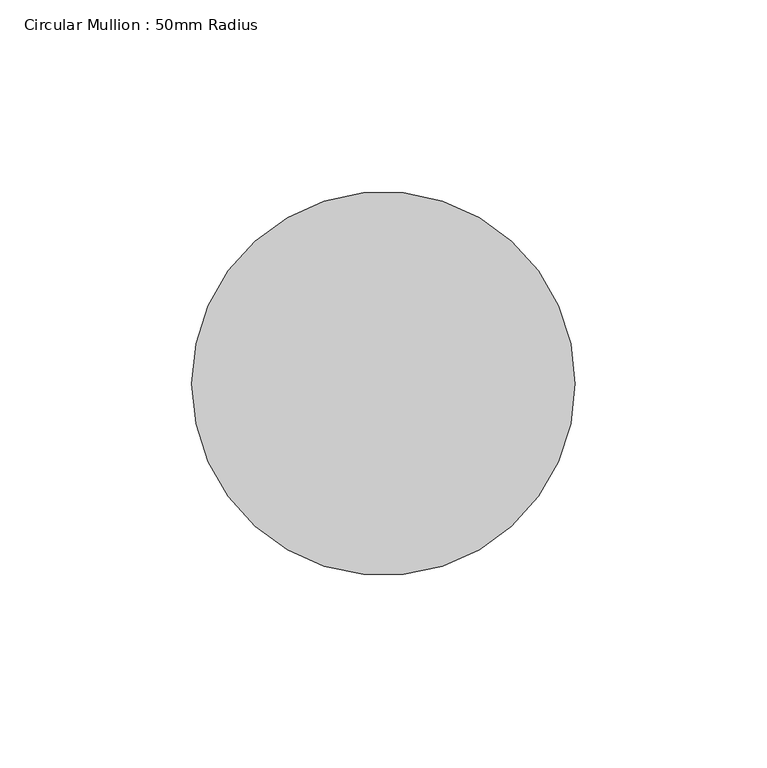
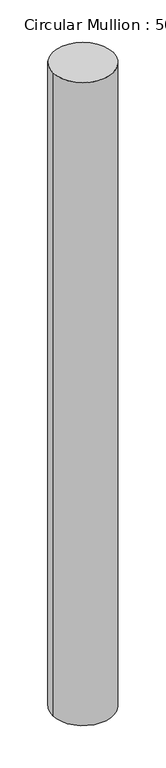
"""IFC4 building model written with IfcOpenShell, lengths in millimetres: member geometry, Circular Mullion : 50mm Radius."""

from ifc_helpers import new_model, si_unit, point, frame, origin, origin_2d, place, context, project, spatial, circle_curve, trimmed, segment, composite_curve, outline, extrude, source, transform, mapped, element, save


def circular_mullion_50mm_radius_a94926c5(model_context):
    return source(origin(), model_context, "Body", "SweptSolid", [
        extrude(outline(composite_curve([segment(trimmed(circle_curve(origin_2d(), 50.0), [point((50.0, 0.0))], [point((-50.0, 0.0))], False, "CARTESIAN"), True, "CONTINUOUS"), segment(trimmed(circle_curve(origin_2d(), 50.0), [point((-50.0, 0.0))], [point((50.0, 0.0))], False, "CARTESIAN"), True, "CONTINUOUS")], self_intersect=False)), frame((0.0, 0.0, -1120.1330061), z_axis=(0.0, 0.0, 1.0), x_axis=(1.0, 0.0, 0.0)), (0.0, 0.0, 1.0), 1120.1330061),
    ])


if __name__ == "__main__":
    model = new_model("IFC4")
    model_context = context("Model", 3, world=origin())
    ifc_project = project(units=[si_unit("LENGTHUNIT", "METRE", prefix="MILLI")], contexts=[model_context])
    site = spatial("IfcSite", under=ifc_project)
    building = spatial("IfcBuilding", under=site)
    placement = place(None, origin())
    circular_mullion_50mm_radius_shape = circular_mullion_50mm_radius_a94926c5(model_context)
    element("IfcMember", 1, ObjectType="Circular Mullion : 50mm Radius", at=placement, inside=building, context=model_context, shape_type="MappedRepresentation", body=[
        mapped(circular_mullion_50mm_radius_shape, transform((0.0, 0.0, 0.0), x_axis=(1.0, 0.0, 0.0), y_axis=(0.0, 1.0, 0.0), z_axis=(0.0, 0.0, 1.0))),
    ])
    save(model, "model.ifc")

# Revit data of these elements
# Type "Circular Mullion : 50mm Radius"
#   built-in parameter 1007350 = 0.164042 (stored number, unit not read)
# Element 1 (IfcMember, "Circular Mullion : 50mm Radius")
#   Materials on its faces: "Aluminium"
# Materials
#   "Aluminium": class "Metal", colour RGB 247 247 247, transparency 0, Description = "Aluminium 6061", Cost = 0
